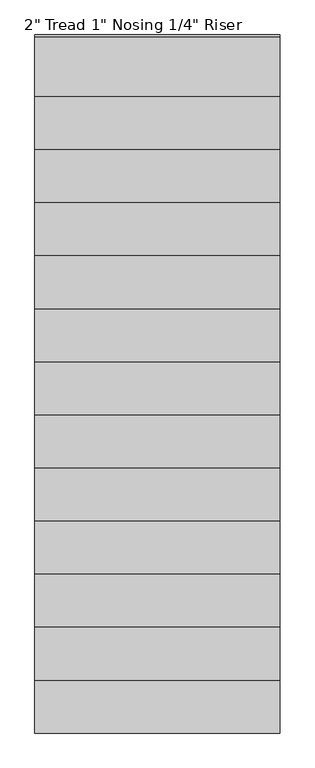
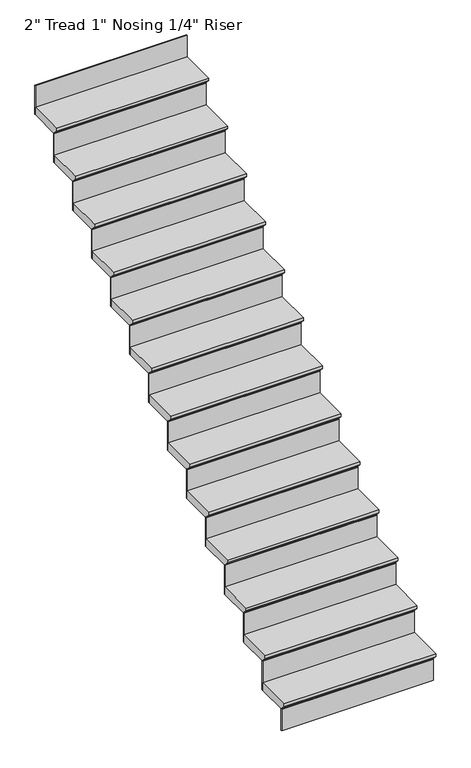
"""IFC4 building model written with IfcOpenShell, lengths in millimetres: stair flight geometry."""

import ifcopenshell
import ifcopenshell.guid

model = None  # the IFC model being written
_history = None  # IfcOwnerHistory: only IFC2X3 demands one
_inside = {}  # id of a spatial element -> (the spatial element, [elements in it])
_under = {}  # id of a project, library or spatial element -> (it, [spatial elements below it])
_declared = {}  # id of a project -> (the project, [libraries it declares])
_typed = {}  # id of a type object -> (the type object, [elements of that type])
_made_of = {}  # id of a material, layer set ... -> (it, [elements and type objects made of it])


def new_model(schema):
    """Start an empty IFC model of exactly this schema.

    Asked for "IFC4X3", IfcOpenShell would pick the latest addendum, in which some entities
    have other attributes; the version numbers below select the first issue.
    IFC2X3 requires an IfcOwnerHistory on every rooted entity: one is made here for all.
    """
    global model, _history
    if schema == "IFC4X3":
        model = ifcopenshell.file(schema_version=(4, 3, 0, 0))
    else:
        model = ifcopenshell.file(schema=schema)
    _inside.clear()
    _under.clear()
    _declared.clear()
    _typed.clear()
    _made_of.clear()
    _history = None
    if model.schema == "IFC2X3":
        org = make("IfcOrganization", Name="unknown")
        user = make(
            "IfcPersonAndOrganization",
            ThePerson=make("IfcPerson", FamilyName="unknown"),
            TheOrganization=org,
        )
        app = make(
            "IfcApplication",
            ApplicationDeveloper=org,
            Version="unknown",
            ApplicationFullName="unknown",
            ApplicationIdentifier="unknown",
        )
        _history = make(
            "IfcOwnerHistory",
            OwningUser=user,
            OwningApplication=app,
            ChangeAction="ADDED",
            CreationDate=0,
        )
    return model


def make(cls, **values):
    """One entity of the class cls with the attributes given. An attribute that is None is left unset."""
    return model.create_entity(
        cls, **{name: value for name, value in values.items() if value is not None}
    )


def rooted(cls, **values):
    """An entity with a GlobalId (a new one), such as an element, a storey or a relation."""
    return make(cls, GlobalId=ifcopenshell.guid.new(), OwnerHistory=_history, **values)


def si_unit(unit_type, name, prefix=None):
    """IfcSIUnit, for example si_unit("LENGTHUNIT", "METRE", prefix="MILLI")."""
    return make("IfcSIUnit", UnitType=unit_type, Prefix=prefix, Name=name)


def assignment(units):
    """IfcUnitAssignment: the units of a project."""
    return None if units is None else make("IfcUnitAssignment", Units=units)


def point(xyz):
    """IfcCartesianPoint."""
    return None if xyz is None else make("IfcCartesianPoint", Coordinates=xyz)


def direction(xyz):
    """IfcDirection."""
    return None if xyz is None else make("IfcDirection", DirectionRatios=xyz)


def frame(location, z_axis=None, x_axis=None):
    """IfcAxis2Placement3D, a coordinate frame: its origin and axes. An axis left out is left unset."""
    return make(
        "IfcAxis2Placement3D",
        Location=point(location),
        Axis=direction(z_axis),
        RefDirection=direction(x_axis),
    )


def origin():
    """The frame at (0, 0, 0) with its axes left unset."""
    return frame((0.0, 0.0, 0.0))


def place(relative_to, where):
    """IfcLocalPlacement: puts the frame where relative to a parent placement (None: the world)."""
    return make(
        "IfcLocalPlacement", PlacementRelTo=relative_to, RelativePlacement=where
    )


def context(
    kind, dimensions, precision=None, world=None, true_north=None, identifier=None
):
    """IfcGeometricRepresentationContext, for example the 3D "Model" context."""
    return make(
        "IfcGeometricRepresentationContext",
        ContextIdentifier=identifier,
        ContextType=kind,
        CoordinateSpaceDimension=dimensions,
        Precision=precision,
        WorldCoordinateSystem=world,
        TrueNorth=true_north,
    )


def project(units=None, contexts=None):
    """IfcProject with its units and contexts."""
    return rooted(
        "IfcProject",
        Name="project",
        RepresentationContexts=contexts,
        UnitsInContext=assignment(units),
    )


def spatial(cls, under=None, at=None, **own):
    """A site, building, storey or space (cls), placed at a placement, below another one or the project."""
    s = rooted(cls, ObjectPlacement=at, **own)
    if under is not None:
        _under.setdefault(under.id(), (under, []))[1].append(s)
    return s


def polyline(points):
    """IfcPolyline through the points."""
    return make("IfcPolyline", Points=[point(p) for p in points])


def outline(outer, holes=None, kind="AREA"):
    """IfcArbitraryClosedProfileDef: a profile drawn as a closed curve; with holes, ...WithVoids."""
    if holes is None:
        return make("IfcArbitraryClosedProfileDef", ProfileType=kind, OuterCurve=outer)
    return make(
        "IfcArbitraryProfileDefWithVoids",
        ProfileType=kind,
        OuterCurve=outer,
        InnerCurves=holes,
    )


def extrude(swept, where, along, depth):
    """IfcExtrudedAreaSolid: the profile swept, set in the frame where, extruded along a direction by depth."""
    return make(
        "IfcExtrudedAreaSolid",
        SweptArea=swept,
        Position=where,
        ExtrudedDirection=direction(along),
        Depth=depth,
    )


def shape(context_of_items, identifier, shape_type, items):
    """IfcShapeRepresentation: the items that make up one representation, for example the "Body"."""
    return make(
        "IfcShapeRepresentation",
        ContextOfItems=context_of_items,
        RepresentationIdentifier=identifier,
        RepresentationType=shape_type,
        Items=items,
    )


def source(mapping_origin, context_of_items, identifier, shape_type, items):
    """IfcRepresentationMap: a shape defined once, which mapped items show again and again."""
    return make(
        "IfcRepresentationMap",
        MappingOrigin=mapping_origin,
        MappedRepresentation=shape(context_of_items, identifier, shape_type, items),
    )


def transform(
    local_origin,
    x_axis=None,
    y_axis=None,
    z_axis=None,
    scale=None,
    scale2=None,
    scale3=None,
    uniform=True,
):
    """IfcCartesianTransformationOperator3D, or its non-uniform kind. x_axis, y_axis, z_axis: its Axis1, 2, 3."""
    if uniform:
        return make(
            "IfcCartesianTransformationOperator3D",
            Axis1=direction(x_axis),
            Axis2=direction(y_axis),
            LocalOrigin=point(local_origin),
            Scale=scale,
            Axis3=direction(z_axis),
        )
    return make(
        "IfcCartesianTransformationOperator3DnonUniform",
        Axis1=direction(x_axis),
        Axis2=direction(y_axis),
        LocalOrigin=point(local_origin),
        Scale=scale,
        Axis3=direction(z_axis),
        Scale2=scale2,
        Scale3=scale3,
    )


def mapped(mapping_source, mapping_target):
    """IfcMappedItem: shows the shape of a source again, moved by a transform."""
    return make(
        "IfcMappedItem", MappingSource=mapping_source, MappingTarget=mapping_target
    )


def made_of(thing, what):
    """Note that an element or type object is made of a material, layer set ...; save() writes the relation."""
    if what is not None:
        _made_of.setdefault(what.id(), (what, []))[1].append(thing)
    return thing


def element(
    cls,
    number,
    at=None,
    inside=None,
    cuts=None,
    type_object=None,
    material=None,
    context=None,
    identifier="Body",
    shape_type=None,
    held_by="IfcProductDefinitionShape",
    body=None,
    shapes=None,
    **own,
):
    """One element of the class cls, such as IfcWall. Its Tag is "e" and its number.

    at: its placement. inside: the storey or other place that contains it. cuts: it is an
    opening in that element (IfcRelVoidsElement). A single representation is given by context,
    identifier, shape_type and body (its items); several are given by shapes. held_by: the class
    of the entity that holds the representations. save() writes the other relations.
    """
    e = rooted(cls, Tag="e%d" % number, ObjectPlacement=at, **own)
    if body is not None:
        shapes = [shape(context, identifier, shape_type, body)]
    if shapes is not None:
        e.Representation = make(held_by, Representations=shapes)
    if inside is not None:
        _inside.setdefault(inside.id(), (inside, []))[1].append(e)
    if cuts is not None:
        rooted(
            "IfcRelVoidsElement", RelatingBuildingElement=cuts, RelatedOpeningElement=e
        )
    if type_object is not None:
        _typed.setdefault(type_object.id(), (type_object, []))[1].append(e)
    return made_of(e, material)


def aggregate(whole, parts):
    """IfcRelAggregates: a whole, such as a stair, and the parts it consists of."""
    return rooted("IfcRelAggregates", RelatingObject=whole, RelatedObjects=parts)


def save(model, path):
    """Write the relations noted so far, then the file.

    IfcRelAggregates (storeys below a building ...), IfcRelContainedInSpatialStructure (elements
    in a storey), IfcRelDefinesByType, IfcRelAssociatesMaterial and IfcRelDeclares: one each for
    every whole, place, type object, material and project.
    """
    for whole, parts in _under.values():
        aggregate(whole, parts)
    for where, things in _inside.values():
        rooted(
            "IfcRelContainedInSpatialStructure",
            RelatedElements=things,
            RelatingStructure=where,
        )
    for kind, things in _typed.values():
        rooted("IfcRelDefinesByType", RelatedObjects=things, RelatingType=kind)
    for what, things in _made_of.values():
        rooted("IfcRelAssociatesMaterial", RelatedObjects=things, RelatingMaterial=what)
    for by, libraries in _declared.values():
        rooted("IfcRelDeclares", RelatingContext=by, RelatedDefinitions=libraries)
    model.write(path)


def stair_flight_b746b64e(model_context):
    return source(origin(), model_context, "Body", "SweptSolid", [
        extrude(outline(polyline([(-2791.5111242, -2476.5), (-2562.9111242, -2476.5), (-2562.9111242, -2527.3), (-2766.1111242, -2527.3), (-2766.1111242, -2520.95), (-2791.5111242, -2495.55), (-2791.5111242, -2476.5)])), frame((-2052.1803068, 0.0, 0.0), z_axis=(1.0, 0.0, 0.0), x_axis=(0.0, 1.0, 0.0)), (0.0, 0.0, 1.0), 939.8),
        extrude(outline(polyline([(-1112.3803068, -2759.7611242), (-1112.3803068, -2766.1111242), (-2052.1803068, -2766.1111242), (-2052.1803068, -2759.7611242), (-1112.3803068, -2759.7611242)])), frame((0.0, 0.0, -2667.0), z_axis=(0.0, 0.0, 1.0), x_axis=(1.0, 0.0, 0.0)), (0.0, 0.0, 1.0), 139.7),
        extrude(outline(polyline([(-1112.3803068, -2556.5611242), (-1112.3803068, -2562.9111242), (-2052.1803068, -2562.9111242), (-2052.1803068, -2556.5611242), (-1112.3803068, -2556.5611242)])), frame((0.0, 0.0, -2527.3), z_axis=(0.0, 0.0, 1.0), x_axis=(1.0, 0.0, 0.0)), (0.0, 0.0, 1.0), 190.5),
        extrude(outline(polyline([(-2588.3111242, -2286.0), (-2359.7111242, -2286.0), (-2359.7111242, -2336.8), (-2562.9111242, -2336.8), (-2562.9111242, -2330.45), (-2588.3111242, -2305.05), (-2588.3111242, -2286.0)])), frame((-2052.1803068, 0.0, 0.0), z_axis=(1.0, 0.0, 0.0), x_axis=(0.0, 1.0, 0.0)), (0.0, 0.0, 1.0), 939.8),
        extrude(outline(polyline([(-1112.3803068, -2353.3611242), (-1112.3803068, -2359.7111242), (-2052.1803068, -2359.7111242), (-2052.1803068, -2353.3611242), (-1112.3803068, -2353.3611242)])), frame((0.0, 0.0, -2336.8), z_axis=(0.0, 0.0, 1.0), x_axis=(1.0, 0.0, 0.0)), (0.0, 0.0, 1.0), 190.5),
        extrude(outline(polyline([(-2385.1111242, -2095.5), (-2156.5111242, -2095.5), (-2156.5111242, -2146.3), (-2359.7111242, -2146.3), (-2359.7111242, -2139.95), (-2385.1111242, -2114.55), (-2385.1111242, -2095.5)])), frame((-2052.1803068, 0.0, 0.0), z_axis=(1.0, 0.0, 0.0), x_axis=(0.0, 1.0, 0.0)), (0.0, 0.0, 1.0), 939.8),
        extrude(outline(polyline([(-1112.3803068, -2150.1611242), (-1112.3803068, -2156.5111242), (-2052.1803068, -2156.5111242), (-2052.1803068, -2150.1611242), (-1112.3803068, -2150.1611242)])), frame((0.0, 0.0, -2146.3), z_axis=(0.0, 0.0, 1.0), x_axis=(1.0, 0.0, 0.0)), (0.0, 0.0, 1.0), 190.5),
        extrude(outline(polyline([(-2181.9111242, -1905.0), (-1953.3111242, -1905.0), (-1953.3111242, -1955.8), (-2156.5111242, -1955.8), (-2156.5111242, -1949.45), (-2181.9111242, -1924.05), (-2181.9111242, -1905.0)])), frame((-2052.1803068, 0.0, 0.0), z_axis=(1.0, 0.0, 0.0), x_axis=(0.0, 1.0, 0.0)), (0.0, 0.0, 1.0), 939.8),
        extrude(outline(polyline([(-1112.3803068, -1946.9611242), (-1112.3803068, -1953.3111242), (-2052.1803068, -1953.3111242), (-2052.1803068, -1946.9611242), (-1112.3803068, -1946.9611242)])), frame((0.0, 0.0, -1955.8), z_axis=(0.0, 0.0, 1.0), x_axis=(1.0, 0.0, 0.0)), (0.0, 0.0, 1.0), 190.5),
        extrude(outline(polyline([(-1978.7111242, -1714.5), (-1750.1111242, -1714.5), (-1750.1111242, -1765.3), (-1953.3111242, -1765.3), (-1953.3111242, -1758.95), (-1978.7111242, -1733.55), (-1978.7111242, -1714.5)])), frame((-2052.1803068, 0.0, 0.0), z_axis=(1.0, 0.0, 0.0), x_axis=(0.0, 1.0, 0.0)), (0.0, 0.0, 1.0), 939.8),
        extrude(outline(polyline([(-1112.3803068, -1743.7611242), (-1112.3803068, -1750.1111242), (-2052.1803068, -1750.1111242), (-2052.1803068, -1743.7611242), (-1112.3803068, -1743.7611242)])), frame((0.0, 0.0, -1765.3), z_axis=(0.0, 0.0, 1.0), x_axis=(1.0, 0.0, 0.0)), (0.0, 0.0, 1.0), 190.5),
        extrude(outline(polyline([(-1775.5111242, -1524.0), (-1546.9111242, -1524.0), (-1546.9111242, -1574.8), (-1750.1111242, -1574.8), (-1750.1111242, -1568.45), (-1775.5111242, -1543.05), (-1775.5111242, -1524.0)])), frame((-2052.1803068, 0.0, 0.0), z_axis=(1.0, 0.0, 0.0), x_axis=(0.0, 1.0, 0.0)), (0.0, 0.0, 1.0), 939.8),
        extrude(outline(polyline([(-1112.3803068, -1540.5611242), (-1112.3803068, -1546.9111242), (-2052.1803068, -1546.9111242), (-2052.1803068, -1540.5611242), (-1112.3803068, -1540.5611242)])), frame((0.0, 0.0, -1574.8), z_axis=(0.0, 0.0, 1.0), x_axis=(1.0, 0.0, 0.0)), (0.0, 0.0, 1.0), 190.5),
        extrude(outline(polyline([(-1572.3111242, -1333.5), (-1343.7111242, -1333.5), (-1343.7111242, -1384.3), (-1546.9111242, -1384.3), (-1546.9111242, -1377.95), (-1572.3111242, -1352.55), (-1572.3111242, -1333.5)])), frame((-2052.1803068, 0.0, 0.0), z_axis=(1.0, 0.0, 0.0), x_axis=(0.0, 1.0, 0.0)), (0.0, 0.0, 1.0), 939.8),
        extrude(outline(polyline([(-1112.3803068, -1337.3611242), (-1112.3803068, -1343.7111242), (-2052.1803068, -1343.7111242), (-2052.1803068, -1337.3611242), (-1112.3803068, -1337.3611242)])), frame((0.0, 0.0, -1384.3), z_axis=(0.0, 0.0, 1.0), x_axis=(1.0, 0.0, 0.0)), (0.0, 0.0, 1.0), 190.5),
        extrude(outline(polyline([(-1369.1111242, -1143.0), (-1140.5111242, -1143.0), (-1140.5111242, -1193.8), (-1343.7111242, -1193.8), (-1343.7111242, -1187.45), (-1369.1111242, -1162.05), (-1369.1111242, -1143.0)])), frame((-2052.1803068, 0.0, 0.0), z_axis=(1.0, 0.0, 0.0), x_axis=(0.0, 1.0, 0.0)), (0.0, 0.0, 1.0), 939.8),
        extrude(outline(polyline([(-1112.3803068, -1134.1611242), (-1112.3803068, -1140.5111242), (-2052.1803068, -1140.5111242), (-2052.1803068, -1134.1611242), (-1112.3803068, -1134.1611242)])), frame((0.0, 0.0, -1193.8), z_axis=(0.0, 0.0, 1.0), x_axis=(1.0, 0.0, 0.0)), (0.0, 0.0, 1.0), 190.5),
        extrude(outline(polyline([(-1165.9111242, -952.5), (-937.3111242, -952.5), (-937.3111242, -1003.3), (-1140.5111242, -1003.3), (-1140.5111242, -996.95), (-1165.9111242, -971.55), (-1165.9111242, -952.5)])), frame((-2052.1803068, 0.0, 0.0), z_axis=(1.0, 0.0, 0.0), x_axis=(0.0, 1.0, 0.0)), (0.0, 0.0, 1.0), 939.8),
        extrude(outline(polyline([(-1112.3803068, -930.9611242), (-1112.3803068, -937.3111242), (-2052.1803068, -937.3111242), (-2052.1803068, -930.9611242), (-1112.3803068, -930.9611242)])), frame((0.0, 0.0, -1003.3), z_axis=(0.0, 0.0, 1.0), x_axis=(1.0, 0.0, 0.0)), (0.0, 0.0, 1.0), 190.5),
        extrude(outline(polyline([(-962.7111242, -762.0), (-734.1111242, -762.0), (-734.1111242, -812.8), (-937.3111242, -812.8), (-937.3111242, -806.45), (-962.7111242, -781.05), (-962.7111242, -762.0)])), frame((-2052.1803068, 0.0, 0.0), z_axis=(1.0, 0.0, 0.0), x_axis=(0.0, 1.0, 0.0)), (0.0, 0.0, 1.0), 939.8),
        extrude(outline(polyline([(-1112.3803068, -727.7611242), (-1112.3803068, -734.1111242), (-2052.1803068, -734.1111242), (-2052.1803068, -727.7611242), (-1112.3803068, -727.7611242)])), frame((0.0, 0.0, -812.8), z_axis=(0.0, 0.0, 1.0), x_axis=(1.0, 0.0, 0.0)), (0.0, 0.0, 1.0), 190.5),
        extrude(outline(polyline([(-759.5111242, -571.5), (-530.9111242, -571.5), (-530.9111242, -622.3), (-734.1111242, -622.3), (-734.1111242, -615.95), (-759.5111242, -590.55), (-759.5111242, -571.5)])), frame((-2052.1803068, 0.0, 0.0), z_axis=(1.0, 0.0, 0.0), x_axis=(0.0, 1.0, 0.0)), (0.0, 0.0, 1.0), 939.8),
        extrude(outline(polyline([(-1112.3803068, -524.5611242), (-1112.3803068, -530.9111242), (-2052.1803068, -530.9111242), (-2052.1803068, -524.5611242), (-1112.3803068, -524.5611242)])), frame((0.0, 0.0, -622.3), z_axis=(0.0, 0.0, 1.0), x_axis=(1.0, 0.0, 0.0)), (0.0, 0.0, 1.0), 190.5),
        extrude(outline(polyline([(-556.3111242, -381.0), (-327.7111242, -381.0), (-327.7111242, -431.8), (-530.9111242, -431.8), (-530.9111242, -425.45), (-556.3111242, -400.05), (-556.3111242, -381.0)])), frame((-2052.1803068, 0.0, 0.0), z_axis=(1.0, 0.0, 0.0), x_axis=(0.0, 1.0, 0.0)), (0.0, 0.0, 1.0), 939.8),
        extrude(outline(polyline([(-1112.3803068, -321.3611242), (-1112.3803068, -327.7111242), (-2052.1803068, -327.7111242), (-2052.1803068, -321.3611242), (-1112.3803068, -321.3611242)])), frame((0.0, 0.0, -431.8), z_axis=(0.0, 0.0, 1.0), x_axis=(1.0, 0.0, 0.0)), (0.0, 0.0, 1.0), 190.5),
        extrude(outline(polyline([(-353.1111242, -190.5), (-124.5111242, -190.5), (-124.5111242, -241.3), (-327.7111242, -241.3), (-327.7111242, -234.95), (-353.1111242, -209.55), (-353.1111242, -190.5)])), frame((-2052.1803068, 0.0, 0.0), z_axis=(1.0, 0.0, 0.0), x_axis=(0.0, 1.0, 0.0)), (0.0, 0.0, 1.0), 939.8),
        extrude(outline(polyline([(-1112.3803068, -118.1611242), (-1112.3803068, -124.5111242), (-2052.1803068, -124.5111242), (-2052.1803068, -118.1611242), (-1112.3803068, -118.1611242)])), frame((0.0, 0.0, -241.3), z_axis=(0.0, 0.0, 1.0), x_axis=(1.0, 0.0, 0.0)), (0.0, 0.0, 1.0), 190.5),
    ])


if __name__ == "__main__":
    model = new_model("IFC4")
    model_context = context("Model", 3, world=origin())
    ifc_project = project(units=[si_unit("LENGTHUNIT", "METRE", prefix="MILLI")], contexts=[model_context])
    site = spatial("IfcSite", under=ifc_project)
    building = spatial("IfcBuilding", under=site)
    placement = place(None, origin())
    stair_flight_shape = stair_flight_b746b64e(model_context)
    element("IfcStairFlight", 1, ObjectType="2\" Tread 1\" Nosing 1/4\" Riser", at=placement, inside=building, context=model_context, shape_type="MappedRepresentation", body=[
        mapped(stair_flight_shape, transform((0.0, 0.0, 0.0), x_axis=(1.0, 0.0, 0.0), y_axis=(0.0, 1.0, 0.0), z_axis=(0.0, 0.0, 1.0))),
    ])
    save(model, "model.ifc")

# Revit data of these elements
# Element 1 (IfcStairFlight, "2\" Tread 1\" Nosing 1/4\" Riser")
#   Materials on its faces: "Oak Flooring"
# Materials
#   "Oak Flooring": class "Wood", colour RGB 216 169 114, transparency 0, Description = "Quercus Rubra", Cost = 0
